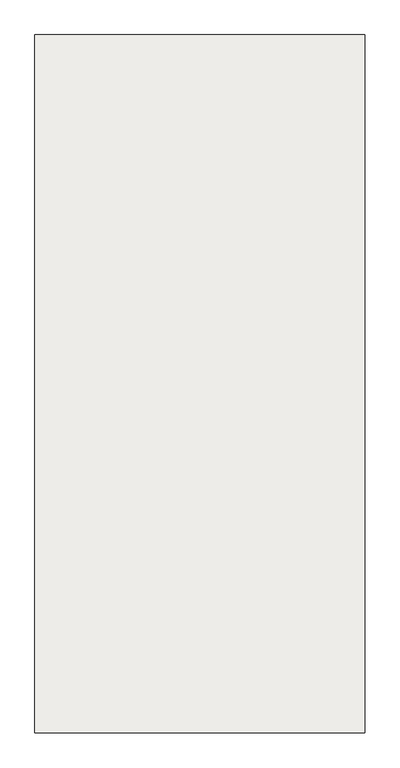
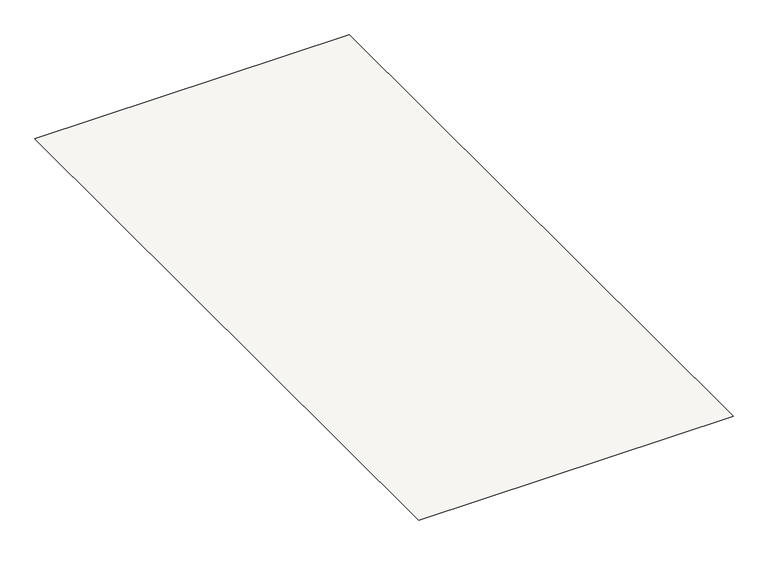
"""IFC4 building model written with IfcOpenShell, lengths in millimetres: slab geometry, EQUIMENT FDN.1 : FTS211_EF_EF1."""

from ifc_helpers import new_model, si_unit, origin, place, context, project, spatial, faceted_brep, source, transform, mapped, element, save


def slab_9a1243d7(model_context):
    return source(origin(), model_context, "Body", "Brep", [
        faceted_brep([(48394.0, 29249.5208589, 199.9720055), (48394.0, 25149.5208589, 199.9720055), (46794.0, 25149.5208589, 199.9720055), (46794.0, 29249.5208589, 199.9720055), (46474.0, 29569.5208589, 399.9720055), (48714.0, 29569.5208589, 399.9720055), (46474.0, 24829.5208589, 399.9720055), (48714.0, 24829.5208589, 399.9720055)], [[[0, 1, 2, 3]], [[0, 3, 4, 5]], [[3, 2, 6, 4]], [[2, 1, 7, 6]], [[1, 0, 5, 7]], [[5, 4, 6, 7]]]),
    ])


if __name__ == "__main__":
    model = new_model("IFC4")
    model_context = context("Model", 3, world=origin())
    ifc_project = project(units=[si_unit("LENGTHUNIT", "METRE", prefix="MILLI")], contexts=[model_context])
    site = spatial("IfcSite", under=ifc_project)
    building = spatial("IfcBuilding", under=site)
    placement = place(None, origin())
    slab_shape = slab_9a1243d7(model_context)
    element("IfcSlab", 1, ObjectType="EQUIMENT FDN.1 : FTS211_EF_EF1", at=placement, inside=building, context=model_context, shape_type="MappedRepresentation", body=[
        mapped(slab_shape, transform((0.0, 0.0, 0.0), x_axis=(1.0, 0.0, 0.0), y_axis=(0.0, 1.0, 0.0), z_axis=(0.0, 0.0, 1.0))),
    ])
    save(model, "model.ifc")

# Revit data of these elements
# Element 1 (IfcSlab, "EQUIMENT FDN.1 : FTS211_EF_EF1")
#   Materials on its faces: "A03AD032-00010_Structural Concrete_UG_20-24MPa"
# Materials
#   "A03AD032-00010_Structural Concrete_UG_20-24MPa": class "Concrete", colour RGB 176 176 176, transparency 0, Keynote = "09910.A1", Description = "Substructure Concrete / Cement Type-1 / 24MPa", Cost = 0
